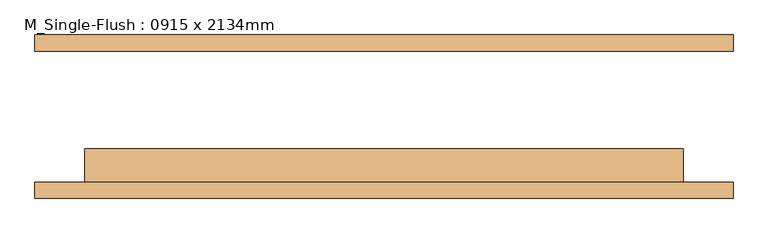
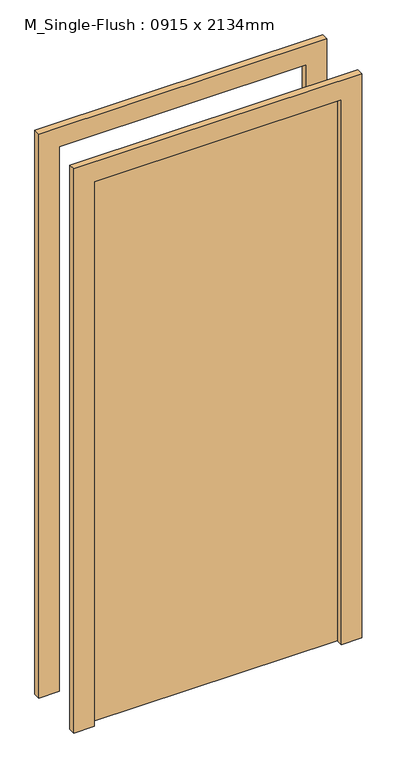
"""IFC4 building model written with IfcOpenShell, lengths in millimetres: door geometry, M_Single-Flush : 0915 x 2134mm."""

import ifcopenshell
import ifcopenshell.guid

model = None  # the IFC model being written
_history = None  # IfcOwnerHistory: only IFC2X3 demands one
_inside = {}  # id of a spatial element -> (the spatial element, [elements in it])
_under = {}  # id of a project, library or spatial element -> (it, [spatial elements below it])
_declared = {}  # id of a project -> (the project, [libraries it declares])
_typed = {}  # id of a type object -> (the type object, [elements of that type])
_made_of = {}  # id of a material, layer set ... -> (it, [elements and type objects made of it])


def new_model(schema):
    """Start an empty IFC model of exactly this schema.

    Asked for "IFC4X3", IfcOpenShell would pick the latest addendum, in which some entities
    have other attributes; the version numbers below select the first issue.
    IFC2X3 requires an IfcOwnerHistory on every rooted entity: one is made here for all.
    """
    global model, _history
    if schema == "IFC4X3":
        model = ifcopenshell.file(schema_version=(4, 3, 0, 0))
    else:
        model = ifcopenshell.file(schema=schema)
    _inside.clear()
    _under.clear()
    _declared.clear()
    _typed.clear()
    _made_of.clear()
    _history = None
    if model.schema == "IFC2X3":
        org = make("IfcOrganization", Name="unknown")
        user = make(
            "IfcPersonAndOrganization",
            ThePerson=make("IfcPerson", FamilyName="unknown"),
            TheOrganization=org,
        )
        app = make(
            "IfcApplication",
            ApplicationDeveloper=org,
            Version="unknown",
            ApplicationFullName="unknown",
            ApplicationIdentifier="unknown",
        )
        _history = make(
            "IfcOwnerHistory",
            OwningUser=user,
            OwningApplication=app,
            ChangeAction="ADDED",
            CreationDate=0,
        )
    return model


def make(cls, **values):
    """One entity of the class cls with the attributes given. An attribute that is None is left unset."""
    return model.create_entity(
        cls, **{name: value for name, value in values.items() if value is not None}
    )


def rooted(cls, **values):
    """An entity with a GlobalId (a new one), such as an element, a storey or a relation."""
    return make(cls, GlobalId=ifcopenshell.guid.new(), OwnerHistory=_history, **values)


def si_unit(unit_type, name, prefix=None):
    """IfcSIUnit, for example si_unit("LENGTHUNIT", "METRE", prefix="MILLI")."""
    return make("IfcSIUnit", UnitType=unit_type, Prefix=prefix, Name=name)


def assignment(units):
    """IfcUnitAssignment: the units of a project."""
    return None if units is None else make("IfcUnitAssignment", Units=units)


def point(xyz):
    """IfcCartesianPoint."""
    return None if xyz is None else make("IfcCartesianPoint", Coordinates=xyz)


def direction(xyz):
    """IfcDirection."""
    return None if xyz is None else make("IfcDirection", DirectionRatios=xyz)


def frame(location, z_axis=None, x_axis=None):
    """IfcAxis2Placement3D, a coordinate frame: its origin and axes. An axis left out is left unset."""
    return make(
        "IfcAxis2Placement3D",
        Location=point(location),
        Axis=direction(z_axis),
        RefDirection=direction(x_axis),
    )


def origin():
    """The frame at (0, 0, 0) with its axes left unset."""
    return frame((0.0, 0.0, 0.0))


def origin_with_axes():
    """The frame at (0, 0, 0) with the z axis (0, 0, 1) and the x axis (1, 0, 0) written out."""
    return frame((0.0, 0.0, 0.0), z_axis=(0.0, 0.0, 1.0), x_axis=(1.0, 0.0, 0.0))


def place(relative_to, where):
    """IfcLocalPlacement: puts the frame where relative to a parent placement (None: the world)."""
    return make(
        "IfcLocalPlacement", PlacementRelTo=relative_to, RelativePlacement=where
    )


def context(
    kind, dimensions, precision=None, world=None, true_north=None, identifier=None
):
    """IfcGeometricRepresentationContext, for example the 3D "Model" context."""
    return make(
        "IfcGeometricRepresentationContext",
        ContextIdentifier=identifier,
        ContextType=kind,
        CoordinateSpaceDimension=dimensions,
        Precision=precision,
        WorldCoordinateSystem=world,
        TrueNorth=true_north,
    )


def project(units=None, contexts=None):
    """IfcProject with its units and contexts."""
    return rooted(
        "IfcProject",
        Name="project",
        RepresentationContexts=contexts,
        UnitsInContext=assignment(units),
    )


def spatial(cls, under=None, at=None, **own):
    """A site, building, storey or space (cls), placed at a placement, below another one or the project."""
    s = rooted(cls, ObjectPlacement=at, **own)
    if under is not None:
        _under.setdefault(under.id(), (under, []))[1].append(s)
    return s


def polyline(points):
    """IfcPolyline through the points."""
    return make("IfcPolyline", Points=[point(p) for p in points])


def outline(outer, holes=None, kind="AREA"):
    """IfcArbitraryClosedProfileDef: a profile drawn as a closed curve; with holes, ...WithVoids."""
    if holes is None:
        return make("IfcArbitraryClosedProfileDef", ProfileType=kind, OuterCurve=outer)
    return make(
        "IfcArbitraryProfileDefWithVoids",
        ProfileType=kind,
        OuterCurve=outer,
        InnerCurves=holes,
    )


def extrude(swept, where, along, depth):
    """IfcExtrudedAreaSolid: the profile swept, set in the frame where, extruded along a direction by depth."""
    return make(
        "IfcExtrudedAreaSolid",
        SweptArea=swept,
        Position=where,
        ExtrudedDirection=direction(along),
        Depth=depth,
    )


def shape(context_of_items, identifier, shape_type, items):
    """IfcShapeRepresentation: the items that make up one representation, for example the "Body"."""
    return make(
        "IfcShapeRepresentation",
        ContextOfItems=context_of_items,
        RepresentationIdentifier=identifier,
        RepresentationType=shape_type,
        Items=items,
    )


def source(mapping_origin, context_of_items, identifier, shape_type, items):
    """IfcRepresentationMap: a shape defined once, which mapped items show again and again."""
    return make(
        "IfcRepresentationMap",
        MappingOrigin=mapping_origin,
        MappedRepresentation=shape(context_of_items, identifier, shape_type, items),
    )


def transform(
    local_origin,
    x_axis=None,
    y_axis=None,
    z_axis=None,
    scale=None,
    scale2=None,
    scale3=None,
    uniform=True,
):
    """IfcCartesianTransformationOperator3D, or its non-uniform kind. x_axis, y_axis, z_axis: its Axis1, 2, 3."""
    if uniform:
        return make(
            "IfcCartesianTransformationOperator3D",
            Axis1=direction(x_axis),
            Axis2=direction(y_axis),
            LocalOrigin=point(local_origin),
            Scale=scale,
            Axis3=direction(z_axis),
        )
    return make(
        "IfcCartesianTransformationOperator3DnonUniform",
        Axis1=direction(x_axis),
        Axis2=direction(y_axis),
        LocalOrigin=point(local_origin),
        Scale=scale,
        Axis3=direction(z_axis),
        Scale2=scale2,
        Scale3=scale3,
    )


def mapped(mapping_source, mapping_target):
    """IfcMappedItem: shows the shape of a source again, moved by a transform."""
    return make(
        "IfcMappedItem", MappingSource=mapping_source, MappingTarget=mapping_target
    )


def made_of(thing, what):
    """Note that an element or type object is made of a material, layer set ...; save() writes the relation."""
    if what is not None:
        _made_of.setdefault(what.id(), (what, []))[1].append(thing)
    return thing


def element(
    cls,
    number,
    at=None,
    inside=None,
    cuts=None,
    type_object=None,
    material=None,
    context=None,
    identifier="Body",
    shape_type=None,
    held_by="IfcProductDefinitionShape",
    body=None,
    shapes=None,
    **own,
):
    """One element of the class cls, such as IfcWall. Its Tag is "e" and its number.

    at: its placement. inside: the storey or other place that contains it. cuts: it is an
    opening in that element (IfcRelVoidsElement). A single representation is given by context,
    identifier, shape_type and body (its items); several are given by shapes. held_by: the class
    of the entity that holds the representations. save() writes the other relations.
    """
    e = rooted(cls, Tag="e%d" % number, ObjectPlacement=at, **own)
    if body is not None:
        shapes = [shape(context, identifier, shape_type, body)]
    if shapes is not None:
        e.Representation = make(held_by, Representations=shapes)
    if inside is not None:
        _inside.setdefault(inside.id(), (inside, []))[1].append(e)
    if cuts is not None:
        rooted(
            "IfcRelVoidsElement", RelatingBuildingElement=cuts, RelatedOpeningElement=e
        )
    if type_object is not None:
        _typed.setdefault(type_object.id(), (type_object, []))[1].append(e)
    return made_of(e, material)


def aggregate(whole, parts):
    """IfcRelAggregates: a whole, such as a stair, and the parts it consists of."""
    return rooted("IfcRelAggregates", RelatingObject=whole, RelatedObjects=parts)


def save(model, path):
    """Write the relations noted so far, then the file.

    IfcRelAggregates (storeys below a building ...), IfcRelContainedInSpatialStructure (elements
    in a storey), IfcRelDefinesByType, IfcRelAssociatesMaterial and IfcRelDeclares: one each for
    every whole, place, type object, material and project.
    """
    for whole, parts in _under.values():
        aggregate(whole, parts)
    for where, things in _inside.values():
        rooted(
            "IfcRelContainedInSpatialStructure",
            RelatedElements=things,
            RelatingStructure=where,
        )
    for kind, things in _typed.values():
        rooted("IfcRelDefinesByType", RelatedObjects=things, RelatingType=kind)
    for what, things in _made_of.values():
        rooted("IfcRelAssociatesMaterial", RelatedObjects=things, RelatingMaterial=what)
    for by, libraries in _declared.values():
        rooted("IfcRelDeclares", RelatingContext=by, RelatedDefinitions=libraries)
    model.write(path)


def m_single_flush_0915_x_2134mm_727434cd(model_context):
    return source(origin(), model_context, "Body", "SweptSolid", [
        extrude(outline(polyline([(2210.0, -533.5), (0.0, -533.5), (0.0, -457.5), (2134.0, -457.5), (2134.0, 457.5), (0.0, 457.5), (0.0, 533.5), (2210.0, 533.5), (2210.0, -533.5)])), frame((0.0, -125.0, 0.0), z_axis=(0.0, 1.0, 0.0), x_axis=(0.0, 0.0, 1.0)), (0.0, 0.0, 1.0), 25.0),
        extrude(outline(polyline([(2210.0, 533.5), (2210.0, -533.5), (0.0, -533.5), (0.0, -457.5), (2134.0, -457.5), (2134.0, 457.5), (0.0, 457.5), (0.0, 533.5), (2210.0, 533.5)])), frame((0.0, 100.0, 0.0), z_axis=(0.0, 1.0, 0.0), x_axis=(0.0, 0.0, 1.0)), (0.0, 0.0, 1.0), 25.0),
        extrude(outline(polyline([(457.5, -49.0), (457.5, -100.0), (-457.5, -100.0), (-457.5, -49.0), (457.5, -49.0)])), origin_with_axes(), (0.0, 0.0, 1.0), 2134.0),
    ])


if __name__ == "__main__":
    model = new_model("IFC4")
    model_context = context("Model", 3, world=origin())
    ifc_project = project(units=[si_unit("LENGTHUNIT", "METRE", prefix="MILLI")], contexts=[model_context])
    site = spatial("IfcSite", under=ifc_project)
    building = spatial("IfcBuilding", under=site)
    placement = place(None, origin())
    m_single_flush_0915_x_2134mm_shape = m_single_flush_0915_x_2134mm_727434cd(model_context)
    element("IfcDoor", 1, ObjectType="M_Single-Flush : 0915 x 2134mm", at=placement, inside=building, context=model_context, shape_type="MappedRepresentation", body=[
        mapped(m_single_flush_0915_x_2134mm_shape, transform((0.0, 0.0, 0.0), x_axis=(1.0, 0.0, 0.0), y_axis=(0.0, 1.0, 0.0), z_axis=(0.0, 0.0, 1.0))),
    ])
    save(model, "model.ifc")

# Revit data of these elements
# Type "M_Single-Flush : 0915 x 2134mm"
#   Type Mark = "15"
#   Construction Type Id = "MDOOR"
#   Analytic Construction = "Metal"
#   Thickness = 0' - 2.00787"
#   Thermal Resistance (R) = 0.270117 (m²·K)/W
#   Heat Transfer Coefficient (U) = 3.7021 W/(m²·K)
#   Height = 7' - 0.01575"
#   Trim Projection Ext = 0' - 0.98425"
#   Trim Projection Int = 0' - 0.98425"
#   Trim Width = 0' - 2.99213"
#   Width = 3' - 0.02362"
#   Door Material = Door - Panel
#   Frame Material = Door - Frame
#   Visual Light Transmittance = 0
#   Solar Heat Gain Coefficient = 0
#   Function = (empty or 0)
#   Wall Closure = (empty or 0)
# Element 1 (IfcDoor, "M_Single-Flush : 0915 x 2134mm")
#   Materials on its faces: "Door - Frame", "Door - Panel"
# Materials
#   "Door - Panel": class "Wood", colour RGB 210 159 95, transparency 0, Cost = 0
#   "Door - Frame": class "Miscellaneous", colour RGB 118 70 51, transparency 0, Cost = 0
